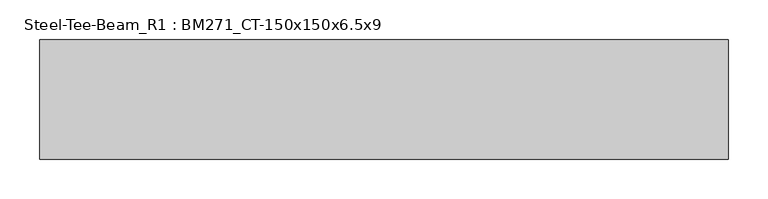
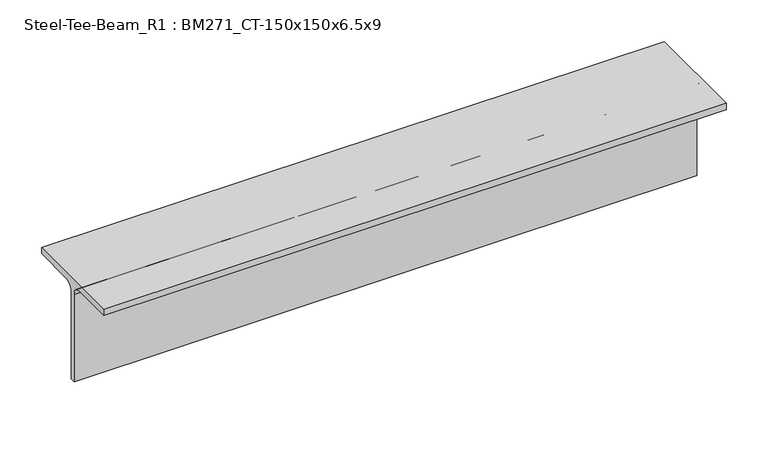
"""IFC4 building model written with IfcOpenShell, lengths in millimetres: member geometry, Steel-Tee-Beam_R1 : BM271_CT-150x150x6.5x9."""

import ifcopenshell
import ifcopenshell.guid

model = None  # the IFC model being written
_history = None  # IfcOwnerHistory: only IFC2X3 demands one
_inside = {}  # id of a spatial element -> (the spatial element, [elements in it])
_under = {}  # id of a project, library or spatial element -> (it, [spatial elements below it])
_declared = {}  # id of a project -> (the project, [libraries it declares])
_typed = {}  # id of a type object -> (the type object, [elements of that type])
_made_of = {}  # id of a material, layer set ... -> (it, [elements and type objects made of it])


def new_model(schema):
    """Start an empty IFC model of exactly this schema.

    Asked for "IFC4X3", IfcOpenShell would pick the latest addendum, in which some entities
    have other attributes; the version numbers below select the first issue.
    IFC2X3 requires an IfcOwnerHistory on every rooted entity: one is made here for all.
    """
    global model, _history
    if schema == "IFC4X3":
        model = ifcopenshell.file(schema_version=(4, 3, 0, 0))
    else:
        model = ifcopenshell.file(schema=schema)
    _inside.clear()
    _under.clear()
    _declared.clear()
    _typed.clear()
    _made_of.clear()
    _history = None
    if model.schema == "IFC2X3":
        org = make("IfcOrganization", Name="unknown")
        user = make(
            "IfcPersonAndOrganization",
            ThePerson=make("IfcPerson", FamilyName="unknown"),
            TheOrganization=org,
        )
        app = make(
            "IfcApplication",
            ApplicationDeveloper=org,
            Version="unknown",
            ApplicationFullName="unknown",
            ApplicationIdentifier="unknown",
        )
        _history = make(
            "IfcOwnerHistory",
            OwningUser=user,
            OwningApplication=app,
            ChangeAction="ADDED",
            CreationDate=0,
        )
    return model


def make(cls, **values):
    """One entity of the class cls with the attributes given. An attribute that is None is left unset."""
    return model.create_entity(
        cls, **{name: value for name, value in values.items() if value is not None}
    )


def rooted(cls, **values):
    """An entity with a GlobalId (a new one), such as an element, a storey or a relation."""
    return make(cls, GlobalId=ifcopenshell.guid.new(), OwnerHistory=_history, **values)


def si_unit(unit_type, name, prefix=None):
    """IfcSIUnit, for example si_unit("LENGTHUNIT", "METRE", prefix="MILLI")."""
    return make("IfcSIUnit", UnitType=unit_type, Prefix=prefix, Name=name)


def assignment(units):
    """IfcUnitAssignment: the units of a project."""
    return None if units is None else make("IfcUnitAssignment", Units=units)


def point(xyz):
    """IfcCartesianPoint."""
    return None if xyz is None else make("IfcCartesianPoint", Coordinates=xyz)


def direction(xyz):
    """IfcDirection."""
    return None if xyz is None else make("IfcDirection", DirectionRatios=xyz)


def frame(location, z_axis=None, x_axis=None):
    """IfcAxis2Placement3D, a coordinate frame: its origin and axes. An axis left out is left unset."""
    return make(
        "IfcAxis2Placement3D",
        Location=point(location),
        Axis=direction(z_axis),
        RefDirection=direction(x_axis),
    )


def frame_2d(location, x_axis=None):
    """IfcAxis2Placement2D, a coordinate frame in the plane: its origin and x axis."""
    return make(
        "IfcAxis2Placement2D", Location=point(location), RefDirection=direction(x_axis)
    )


def origin():
    """The frame at (0, 0, 0) with its axes left unset."""
    return frame((0.0, 0.0, 0.0))


def place(relative_to, where):
    """IfcLocalPlacement: puts the frame where relative to a parent placement (None: the world)."""
    return make(
        "IfcLocalPlacement", PlacementRelTo=relative_to, RelativePlacement=where
    )


def context(
    kind, dimensions, precision=None, world=None, true_north=None, identifier=None
):
    """IfcGeometricRepresentationContext, for example the 3D "Model" context."""
    return make(
        "IfcGeometricRepresentationContext",
        ContextIdentifier=identifier,
        ContextType=kind,
        CoordinateSpaceDimension=dimensions,
        Precision=precision,
        WorldCoordinateSystem=world,
        TrueNorth=true_north,
    )


def project(units=None, contexts=None):
    """IfcProject with its units and contexts."""
    return rooted(
        "IfcProject",
        Name="project",
        RepresentationContexts=contexts,
        UnitsInContext=assignment(units),
    )


def spatial(cls, under=None, at=None, **own):
    """A site, building, storey or space (cls), placed at a placement, below another one or the project."""
    s = rooted(cls, ObjectPlacement=at, **own)
    if under is not None:
        _under.setdefault(under.id(), (under, []))[1].append(s)
    return s


def polyline(points):
    """IfcPolyline through the points."""
    return make("IfcPolyline", Points=[point(p) for p in points])


def circle_curve(where, radius):
    """IfcCircle in the frame where."""
    return make("IfcCircle", Position=where, Radius=radius)


def trimmed(basis, trim1, trim2, sense, master):
    """IfcTrimmedCurve: the piece of a basis curve between two trims."""
    return make(
        "IfcTrimmedCurve",
        BasisCurve=basis,
        Trim1=trim1,
        Trim2=trim2,
        SenseAgreement=sense,
        MasterRepresentation=master,
    )


def segment(curve, same_sense, transition):
    """IfcCompositeCurveSegment."""
    return make(
        "IfcCompositeCurveSegment",
        Transition=transition,
        SameSense=same_sense,
        ParentCurve=curve,
    )


def composite_curve(segments, self_intersect=None):
    """IfcCompositeCurve: segments joined end to end."""
    return make("IfcCompositeCurve", Segments=segments, SelfIntersect=self_intersect)


def outline(outer, holes=None, kind="AREA"):
    """IfcArbitraryClosedProfileDef: a profile drawn as a closed curve; with holes, ...WithVoids."""
    if holes is None:
        return make("IfcArbitraryClosedProfileDef", ProfileType=kind, OuterCurve=outer)
    return make(
        "IfcArbitraryProfileDefWithVoids",
        ProfileType=kind,
        OuterCurve=outer,
        InnerCurves=holes,
    )


def extrude(swept, where, along, depth):
    """IfcExtrudedAreaSolid: the profile swept, set in the frame where, extruded along a direction by depth."""
    return make(
        "IfcExtrudedAreaSolid",
        SweptArea=swept,
        Position=where,
        ExtrudedDirection=direction(along),
        Depth=depth,
    )


def shape(context_of_items, identifier, shape_type, items):
    """IfcShapeRepresentation: the items that make up one representation, for example the "Body"."""
    return make(
        "IfcShapeRepresentation",
        ContextOfItems=context_of_items,
        RepresentationIdentifier=identifier,
        RepresentationType=shape_type,
        Items=items,
    )


def source(mapping_origin, context_of_items, identifier, shape_type, items):
    """IfcRepresentationMap: a shape defined once, which mapped items show again and again."""
    return make(
        "IfcRepresentationMap",
        MappingOrigin=mapping_origin,
        MappedRepresentation=shape(context_of_items, identifier, shape_type, items),
    )


def transform(
    local_origin,
    x_axis=None,
    y_axis=None,
    z_axis=None,
    scale=None,
    scale2=None,
    scale3=None,
    uniform=True,
):
    """IfcCartesianTransformationOperator3D, or its non-uniform kind. x_axis, y_axis, z_axis: its Axis1, 2, 3."""
    if uniform:
        return make(
            "IfcCartesianTransformationOperator3D",
            Axis1=direction(x_axis),
            Axis2=direction(y_axis),
            LocalOrigin=point(local_origin),
            Scale=scale,
            Axis3=direction(z_axis),
        )
    return make(
        "IfcCartesianTransformationOperator3DnonUniform",
        Axis1=direction(x_axis),
        Axis2=direction(y_axis),
        LocalOrigin=point(local_origin),
        Scale=scale,
        Axis3=direction(z_axis),
        Scale2=scale2,
        Scale3=scale3,
    )


def mapped(mapping_source, mapping_target):
    """IfcMappedItem: shows the shape of a source again, moved by a transform."""
    return make(
        "IfcMappedItem", MappingSource=mapping_source, MappingTarget=mapping_target
    )


def made_of(thing, what):
    """Note that an element or type object is made of a material, layer set ...; save() writes the relation."""
    if what is not None:
        _made_of.setdefault(what.id(), (what, []))[1].append(thing)
    return thing


def element(
    cls,
    number,
    at=None,
    inside=None,
    cuts=None,
    type_object=None,
    material=None,
    context=None,
    identifier="Body",
    shape_type=None,
    held_by="IfcProductDefinitionShape",
    body=None,
    shapes=None,
    **own,
):
    """One element of the class cls, such as IfcWall. Its Tag is "e" and its number.

    at: its placement. inside: the storey or other place that contains it. cuts: it is an
    opening in that element (IfcRelVoidsElement). A single representation is given by context,
    identifier, shape_type and body (its items); several are given by shapes. held_by: the class
    of the entity that holds the representations. save() writes the other relations.
    """
    e = rooted(cls, Tag="e%d" % number, ObjectPlacement=at, **own)
    if body is not None:
        shapes = [shape(context, identifier, shape_type, body)]
    if shapes is not None:
        e.Representation = make(held_by, Representations=shapes)
    if inside is not None:
        _inside.setdefault(inside.id(), (inside, []))[1].append(e)
    if cuts is not None:
        rooted(
            "IfcRelVoidsElement", RelatingBuildingElement=cuts, RelatedOpeningElement=e
        )
    if type_object is not None:
        _typed.setdefault(type_object.id(), (type_object, []))[1].append(e)
    return made_of(e, material)


def aggregate(whole, parts):
    """IfcRelAggregates: a whole, such as a stair, and the parts it consists of."""
    return rooted("IfcRelAggregates", RelatingObject=whole, RelatedObjects=parts)


def save(model, path):
    """Write the relations noted so far, then the file.

    IfcRelAggregates (storeys below a building ...), IfcRelContainedInSpatialStructure (elements
    in a storey), IfcRelDefinesByType, IfcRelAssociatesMaterial and IfcRelDeclares: one each for
    every whole, place, type object, material and project.
    """
    for whole, parts in _under.values():
        aggregate(whole, parts)
    for where, things in _inside.values():
        rooted(
            "IfcRelContainedInSpatialStructure",
            RelatedElements=things,
            RelatingStructure=where,
        )
    for kind, things in _typed.values():
        rooted("IfcRelDefinesByType", RelatedObjects=things, RelatingType=kind)
    for what, things in _made_of.values():
        rooted("IfcRelAssociatesMaterial", RelatedObjects=things, RelatingMaterial=what)
    for by, libraries in _declared.values():
        rooted("IfcRelDeclares", RelatingContext=by, RelatedDefinitions=libraries)
    model.write(path)


def steel_tee_beam_r1_bm271_ct_150x150x6_5x9_73514d7c(model_context):
    return source(origin(), model_context, "Body", "SweptSolid", [
        extrude(outline(composite_curve([segment(polyline([(-75.0, 75.0), (75.0, 75.0), (75.0, 66.0), (16.25, 66.0)]), True, "CONTINUOUS"), segment(trimmed(circle_curve(frame_2d((16.25, 53.0)), 13.0), [point((16.25, 66.0))], [point((3.25, 53.0))], True, "CARTESIAN"), True, "CONTINUOUS"), segment(polyline([(3.25, 53.0), (3.25, -75.0), (-3.25, -75.0), (-3.25, 53.0)]), True, "CONTINUOUS"), segment(trimmed(circle_curve(frame_2d((-16.25, 53.0)), 13.0), [point((-3.25, 53.0))], [point((-16.25, 66.0))], True, "CARTESIAN"), True, "CONTINUOUS"), segment(polyline([(-16.25, 66.0), (-75.0, 66.0), (-75.0, 75.0)]), True, "CONTINUOUS")], self_intersect=False)), frame((-365.9474508, 0.0, 0.0), z_axis=(1.0, 0.0, 0.0), x_axis=(0.0, 1.0, 0.0)), (0.0, 0.0, 1.0), 865.9474508),
    ])


if __name__ == "__main__":
    model = new_model("IFC4")
    model_context = context("Model", 3, world=origin())
    ifc_project = project(units=[si_unit("LENGTHUNIT", "METRE", prefix="MILLI")], contexts=[model_context])
    site = spatial("IfcSite", under=ifc_project)
    building = spatial("IfcBuilding", under=site)
    placement = place(None, origin())
    steel_tee_beam_r1_bm271_ct_150x150x6_5x9_shape = steel_tee_beam_r1_bm271_ct_150x150x6_5x9_73514d7c(model_context)
    element("IfcMember", 1, ObjectType="Steel-Tee-Beam_R1 : BM271_CT-150x150x6.5x9", at=placement, inside=building, context=model_context, shape_type="MappedRepresentation", body=[
        mapped(steel_tee_beam_r1_bm271_ct_150x150x6_5x9_shape, transform((0.0, 0.0, 0.0), x_axis=(1.0, 0.0, 0.0), y_axis=(0.0, 1.0, 0.0), z_axis=(0.0, 0.0, 1.0))),
    ])
    save(model, "model.ifc")

# Revit data of these elements
# Type "Steel-Tee-Beam_R1 : BM271_CT-150x150x6.5x9"
#   Keynote = "CT-150x150x6.5x9"
#   Surface Area = 0.588841 m²/m
#   Section Area = 23.3904 cm²
#   Mass per Unit Length = 18.3614 kg/m
#   Length [instance default] = 1.5240 m
#   bf = 0.1500 m
#   d = 0.1500 m
#   k = 0.0220 m
#   r = 0.0130 m
#   tf = 0.0090 m
#   tw = 0.0065 m
#   hec_material4 [instance default] = none
#   hec_material3 [instance default] = none
#   hec_material2 [instance default] = none
#   hec_material1 [instance default] = none
#   Structural Material [instance default] = Steel, 45-345
#   Assembly Code = ""
# Element 1 (IfcMember, "Steel-Tee-Beam_R1 : BM271_CT-150x150x6.5x9")
#   Structural Material = none
# Materials
#   "Steel, 45-345": class "Metal", colour RGB 189 187 185, transparency 0, Description = "Steel 345 MPa", Cost = 0
